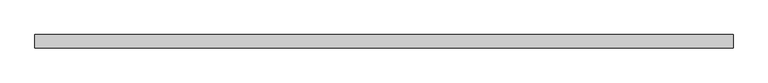
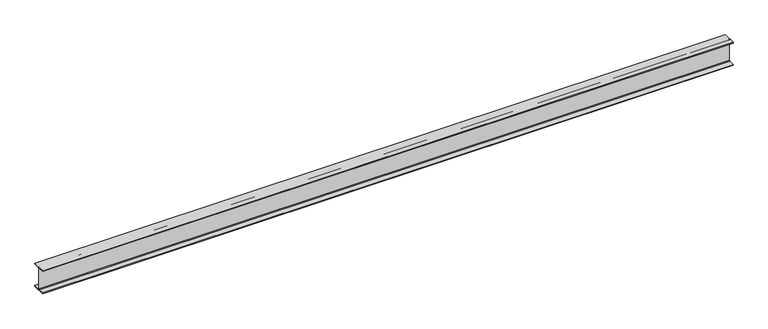
"""IFC4 building model written with IfcOpenShell, lengths in millimetres: beam geometry, Old_Steel Beam_H-KSD3502 : H_SB_ASB_H-350×175x7x11."""

from ifc_helpers import new_model, si_unit, point, frame, frame_2d, origin, place, context, project, spatial, polyline, circle_curve, trimmed, segment, composite_curve, outline, extrude, source, transform, mapped, element, save


def beam_e21a578f(model_context):
    return source(origin(), model_context, "Body", "SweptSolid", [
        extrude(outline(composite_curve([segment(polyline([(82.5, -141.5), (82.5, -151.7), (-82.5, -151.7), (-82.5, -141.5), (-11.9, -141.5)]), True, "CONTINUOUS"), segment(trimmed(circle_curve(frame_2d((-11.9, -132.6)), 8.9), [point((-11.9, -141.5))], [point((-3.0, -132.6))], True, "CARTESIAN"), True, "CONTINUOUS"), segment(polyline([(-3.0, -132.6), (-3.0, 132.6)]), True, "CONTINUOUS"), segment(trimmed(circle_curve(frame_2d((-11.9, 132.6)), 8.9), [point((-3.0, 132.6))], [point((-11.9, 141.5))], True, "CARTESIAN"), True, "CONTINUOUS"), segment(polyline([(-11.9, 141.5), (-82.5, 141.5), (-82.5, 151.7), (82.5, 151.7), (82.5, 141.5), (11.9, 141.5)]), True, "CONTINUOUS"), segment(trimmed(circle_curve(frame_2d((11.9, 132.6)), 8.9), [point((11.9, 141.5))], [point((3.0, 132.6))], True, "CARTESIAN"), True, "CONTINUOUS"), segment(polyline([(3.0, 132.6), (3.0, -132.6)]), True, "CONTINUOUS"), segment(trimmed(circle_curve(frame_2d((11.9, -132.6)), 8.9), [point((3.0, -132.6))], [point((11.9, -141.5))], True, "CARTESIAN"), True, "CONTINUOUS"), segment(polyline([(11.9, -141.5), (82.5, -141.5)]), True, "CONTINUOUS")], self_intersect=False)), frame((-4333.8712061, 0.0, 0.0), z_axis=(1.0, 0.0, 0.0), x_axis=(0.0, 1.0, 0.0)), (0.0, 0.0, 1.0), 8632.7424123),
    ])


if __name__ == "__main__":
    model = new_model("IFC4")
    model_context = context("Model", 3, world=origin())
    ifc_project = project(units=[si_unit("LENGTHUNIT", "METRE", prefix="MILLI")], contexts=[model_context])
    site = spatial("IfcSite", under=ifc_project)
    building = spatial("IfcBuilding", under=site)
    placement = place(None, origin())
    beam_shape = beam_e21a578f(model_context)
    element("IfcBeam", 1, ObjectType="Old_Steel Beam_H-KSD3502 : H_SB_ASB_H-350×175x7x11", at=placement, inside=building, context=model_context, shape_type="MappedRepresentation", body=[
        mapped(beam_shape, transform((0.0, 0.0, 0.0), x_axis=(1.0, 0.0, 0.0), y_axis=(0.0, 1.0, 0.0), z_axis=(0.0, 0.0, 1.0))),
    ])
    save(model, "model.ifc")

# Revit data of these elements
# Type "Old_Steel Beam_H-KSD3502 : H_SB_ASB_H-350×175x7x11"
#   Width = 17.5 cm
#   Web Thickness = 0.7 cm
#   Web Fillet = 1.4 cm
#   Warping Constant = 282290.0 cm⁶
#   Torsional Moment of Inertia = 19.4042 cm⁴
#   Torsional Modulus = 1.0 cm³
#   Section Area = 63.14 cm²
#   Plastic Modulus weak axis = 174.0 cm³
#   Plastic Modulus strong axis = 868.0 cm³
#   Perimeter = 1.36 m²/m
#   Nominal Weight = 49.60 kgf/m
#   Moment of Inertia weak axis = 984.00 cm⁴
#   Moment of Inertia strong axis = 13600.00 cm⁴
#   Height = 35.0 cm
#   Flange Thickness = 1.1 cm
#   Elastic Modulus weak axis = 112.0 cm³
#   Elastic Modulus strong axis = 775.0 cm³
#   Centroid Vertical = 17.5 cm
#   Centroid Horizontal = 8.75 cm
#   Length [instance default] = 1.5240 m
#   Structural Material [instance default] = Steel, 45-345
#   Assembly Code = ""
# Element 1 (IfcBeam, "Old_Steel Beam_H-KSD3502 : H_SB_ASB_H-350×175x7x11")
#   Structural Material = none
# Materials
#   "Steel, 45-345": class "Metal", colour RGB 189 187 185, transparency 0, Description = "Steel 345 MPa", Cost = 0
